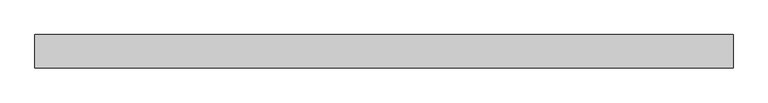
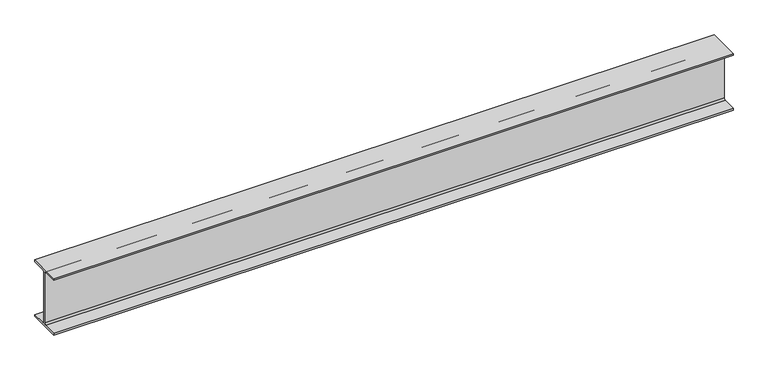
"""IFC4 building model written with IfcOpenShell, lengths in millimetres: beam geometry, Steel Beam_H-KSD3502 : H_SB_ASB_H-200x200x8x12."""

import ifcopenshell
import ifcopenshell.guid

model = None  # the IFC model being written
_history = None  # IfcOwnerHistory: only IFC2X3 demands one
_inside = {}  # id of a spatial element -> (the spatial element, [elements in it])
_under = {}  # id of a project, library or spatial element -> (it, [spatial elements below it])
_declared = {}  # id of a project -> (the project, [libraries it declares])
_typed = {}  # id of a type object -> (the type object, [elements of that type])
_made_of = {}  # id of a material, layer set ... -> (it, [elements and type objects made of it])


def new_model(schema):
    """Start an empty IFC model of exactly this schema.

    Asked for "IFC4X3", IfcOpenShell would pick the latest addendum, in which some entities
    have other attributes; the version numbers below select the first issue.
    IFC2X3 requires an IfcOwnerHistory on every rooted entity: one is made here for all.
    """
    global model, _history
    if schema == "IFC4X3":
        model = ifcopenshell.file(schema_version=(4, 3, 0, 0))
    else:
        model = ifcopenshell.file(schema=schema)
    _inside.clear()
    _under.clear()
    _declared.clear()
    _typed.clear()
    _made_of.clear()
    _history = None
    if model.schema == "IFC2X3":
        org = make("IfcOrganization", Name="unknown")
        user = make(
            "IfcPersonAndOrganization",
            ThePerson=make("IfcPerson", FamilyName="unknown"),
            TheOrganization=org,
        )
        app = make(
            "IfcApplication",
            ApplicationDeveloper=org,
            Version="unknown",
            ApplicationFullName="unknown",
            ApplicationIdentifier="unknown",
        )
        _history = make(
            "IfcOwnerHistory",
            OwningUser=user,
            OwningApplication=app,
            ChangeAction="ADDED",
            CreationDate=0,
        )
    return model


def make(cls, **values):
    """One entity of the class cls with the attributes given. An attribute that is None is left unset."""
    return model.create_entity(
        cls, **{name: value for name, value in values.items() if value is not None}
    )


def rooted(cls, **values):
    """An entity with a GlobalId (a new one), such as an element, a storey or a relation."""
    return make(cls, GlobalId=ifcopenshell.guid.new(), OwnerHistory=_history, **values)


def si_unit(unit_type, name, prefix=None):
    """IfcSIUnit, for example si_unit("LENGTHUNIT", "METRE", prefix="MILLI")."""
    return make("IfcSIUnit", UnitType=unit_type, Prefix=prefix, Name=name)


def assignment(units):
    """IfcUnitAssignment: the units of a project."""
    return None if units is None else make("IfcUnitAssignment", Units=units)


def point(xyz):
    """IfcCartesianPoint."""
    return None if xyz is None else make("IfcCartesianPoint", Coordinates=xyz)


def direction(xyz):
    """IfcDirection."""
    return None if xyz is None else make("IfcDirection", DirectionRatios=xyz)


def frame(location, z_axis=None, x_axis=None):
    """IfcAxis2Placement3D, a coordinate frame: its origin and axes. An axis left out is left unset."""
    return make(
        "IfcAxis2Placement3D",
        Location=point(location),
        Axis=direction(z_axis),
        RefDirection=direction(x_axis),
    )


def frame_2d(location, x_axis=None):
    """IfcAxis2Placement2D, a coordinate frame in the plane: its origin and x axis."""
    return make(
        "IfcAxis2Placement2D", Location=point(location), RefDirection=direction(x_axis)
    )


def origin():
    """The frame at (0, 0, 0) with its axes left unset."""
    return frame((0.0, 0.0, 0.0))


def place(relative_to, where):
    """IfcLocalPlacement: puts the frame where relative to a parent placement (None: the world)."""
    return make(
        "IfcLocalPlacement", PlacementRelTo=relative_to, RelativePlacement=where
    )


def context(
    kind, dimensions, precision=None, world=None, true_north=None, identifier=None
):
    """IfcGeometricRepresentationContext, for example the 3D "Model" context."""
    return make(
        "IfcGeometricRepresentationContext",
        ContextIdentifier=identifier,
        ContextType=kind,
        CoordinateSpaceDimension=dimensions,
        Precision=precision,
        WorldCoordinateSystem=world,
        TrueNorth=true_north,
    )


def project(units=None, contexts=None):
    """IfcProject with its units and contexts."""
    return rooted(
        "IfcProject",
        Name="project",
        RepresentationContexts=contexts,
        UnitsInContext=assignment(units),
    )


def spatial(cls, under=None, at=None, **own):
    """A site, building, storey or space (cls), placed at a placement, below another one or the project."""
    s = rooted(cls, ObjectPlacement=at, **own)
    if under is not None:
        _under.setdefault(under.id(), (under, []))[1].append(s)
    return s


def polyline(points):
    """IfcPolyline through the points."""
    return make("IfcPolyline", Points=[point(p) for p in points])


def circle_curve(where, radius):
    """IfcCircle in the frame where."""
    return make("IfcCircle", Position=where, Radius=radius)


def trimmed(basis, trim1, trim2, sense, master):
    """IfcTrimmedCurve: the piece of a basis curve between two trims."""
    return make(
        "IfcTrimmedCurve",
        BasisCurve=basis,
        Trim1=trim1,
        Trim2=trim2,
        SenseAgreement=sense,
        MasterRepresentation=master,
    )


def segment(curve, same_sense, transition):
    """IfcCompositeCurveSegment."""
    return make(
        "IfcCompositeCurveSegment",
        Transition=transition,
        SameSense=same_sense,
        ParentCurve=curve,
    )


def composite_curve(segments, self_intersect=None):
    """IfcCompositeCurve: segments joined end to end."""
    return make("IfcCompositeCurve", Segments=segments, SelfIntersect=self_intersect)


def outline(outer, holes=None, kind="AREA"):
    """IfcArbitraryClosedProfileDef: a profile drawn as a closed curve; with holes, ...WithVoids."""
    if holes is None:
        return make("IfcArbitraryClosedProfileDef", ProfileType=kind, OuterCurve=outer)
    return make(
        "IfcArbitraryProfileDefWithVoids",
        ProfileType=kind,
        OuterCurve=outer,
        InnerCurves=holes,
    )


def extrude(swept, where, along, depth):
    """IfcExtrudedAreaSolid: the profile swept, set in the frame where, extruded along a direction by depth."""
    return make(
        "IfcExtrudedAreaSolid",
        SweptArea=swept,
        Position=where,
        ExtrudedDirection=direction(along),
        Depth=depth,
    )


def shape(context_of_items, identifier, shape_type, items):
    """IfcShapeRepresentation: the items that make up one representation, for example the "Body"."""
    return make(
        "IfcShapeRepresentation",
        ContextOfItems=context_of_items,
        RepresentationIdentifier=identifier,
        RepresentationType=shape_type,
        Items=items,
    )


def source(mapping_origin, context_of_items, identifier, shape_type, items):
    """IfcRepresentationMap: a shape defined once, which mapped items show again and again."""
    return make(
        "IfcRepresentationMap",
        MappingOrigin=mapping_origin,
        MappedRepresentation=shape(context_of_items, identifier, shape_type, items),
    )


def transform(
    local_origin,
    x_axis=None,
    y_axis=None,
    z_axis=None,
    scale=None,
    scale2=None,
    scale3=None,
    uniform=True,
):
    """IfcCartesianTransformationOperator3D, or its non-uniform kind. x_axis, y_axis, z_axis: its Axis1, 2, 3."""
    if uniform:
        return make(
            "IfcCartesianTransformationOperator3D",
            Axis1=direction(x_axis),
            Axis2=direction(y_axis),
            LocalOrigin=point(local_origin),
            Scale=scale,
            Axis3=direction(z_axis),
        )
    return make(
        "IfcCartesianTransformationOperator3DnonUniform",
        Axis1=direction(x_axis),
        Axis2=direction(y_axis),
        LocalOrigin=point(local_origin),
        Scale=scale,
        Axis3=direction(z_axis),
        Scale2=scale2,
        Scale3=scale3,
    )


def mapped(mapping_source, mapping_target):
    """IfcMappedItem: shows the shape of a source again, moved by a transform."""
    return make(
        "IfcMappedItem", MappingSource=mapping_source, MappingTarget=mapping_target
    )


def made_of(thing, what):
    """Note that an element or type object is made of a material, layer set ...; save() writes the relation."""
    if what is not None:
        _made_of.setdefault(what.id(), (what, []))[1].append(thing)
    return thing


def element(
    cls,
    number,
    at=None,
    inside=None,
    cuts=None,
    type_object=None,
    material=None,
    context=None,
    identifier="Body",
    shape_type=None,
    held_by="IfcProductDefinitionShape",
    body=None,
    shapes=None,
    **own,
):
    """One element of the class cls, such as IfcWall. Its Tag is "e" and its number.

    at: its placement. inside: the storey or other place that contains it. cuts: it is an
    opening in that element (IfcRelVoidsElement). A single representation is given by context,
    identifier, shape_type and body (its items); several are given by shapes. held_by: the class
    of the entity that holds the representations. save() writes the other relations.
    """
    e = rooted(cls, Tag="e%d" % number, ObjectPlacement=at, **own)
    if body is not None:
        shapes = [shape(context, identifier, shape_type, body)]
    if shapes is not None:
        e.Representation = make(held_by, Representations=shapes)
    if inside is not None:
        _inside.setdefault(inside.id(), (inside, []))[1].append(e)
    if cuts is not None:
        rooted(
            "IfcRelVoidsElement", RelatingBuildingElement=cuts, RelatedOpeningElement=e
        )
    if type_object is not None:
        _typed.setdefault(type_object.id(), (type_object, []))[1].append(e)
    return made_of(e, material)


def aggregate(whole, parts):
    """IfcRelAggregates: a whole, such as a stair, and the parts it consists of."""
    return rooted("IfcRelAggregates", RelatingObject=whole, RelatedObjects=parts)


def save(model, path):
    """Write the relations noted so far, then the file.

    IfcRelAggregates (storeys below a building ...), IfcRelContainedInSpatialStructure (elements
    in a storey), IfcRelDefinesByType, IfcRelAssociatesMaterial and IfcRelDeclares: one each for
    every whole, place, type object, material and project.
    """
    for whole, parts in _under.values():
        aggregate(whole, parts)
    for where, things in _inside.values():
        rooted(
            "IfcRelContainedInSpatialStructure",
            RelatedElements=things,
            RelatingStructure=where,
        )
    for kind, things in _typed.values():
        rooted("IfcRelDefinesByType", RelatedObjects=things, RelatingType=kind)
    for what, things in _made_of.values():
        rooted("IfcRelAssociatesMaterial", RelatedObjects=things, RelatingMaterial=what)
    for by, libraries in _declared.values():
        rooted("IfcRelDeclares", RelatingContext=by, RelatedDefinitions=libraries)
    model.write(path)


def beam_b71a2e39(model_context):
    return source(origin(), model_context, "Body", "SweptSolid", [
        extrude(outline(composite_curve([segment(polyline([(82.5, -141.5), (82.5, -151.7), (-82.5, -151.7), (-82.5, -141.5), (-11.9, -141.5)]), True, "CONTINUOUS"), segment(trimmed(circle_curve(frame_2d((-11.9, -132.6)), 8.9), [point((-11.9, -141.5))], [point((-3.0, -132.6))], True, "CARTESIAN"), True, "CONTINUOUS"), segment(polyline([(-3.0, -132.6), (-3.0, 132.6)]), True, "CONTINUOUS"), segment(trimmed(circle_curve(frame_2d((-11.9, 132.6)), 8.9), [point((-3.0, 132.6))], [point((-11.9, 141.5))], True, "CARTESIAN"), True, "CONTINUOUS"), segment(polyline([(-11.9, 141.5), (-82.5, 141.5), (-82.5, 151.7), (82.5, 151.7), (82.5, 141.5), (11.9, 141.5)]), True, "CONTINUOUS"), segment(trimmed(circle_curve(frame_2d((11.9, 132.6)), 8.9), [point((11.9, 141.5))], [point((3.0, 132.6))], True, "CARTESIAN"), True, "CONTINUOUS"), segment(polyline([(3.0, 132.6), (3.0, -132.6)]), True, "CONTINUOUS"), segment(trimmed(circle_curve(frame_2d((11.9, -132.6)), 8.9), [point((3.0, -132.6))], [point((11.9, -141.5))], True, "CARTESIAN"), True, "CONTINUOUS"), segment(polyline([(11.9, -141.5), (82.5, -141.5)]), True, "CONTINUOUS")], self_intersect=False)), frame((-1683.7594404, 0.0, 0.0), z_axis=(1.0, 0.0, 0.0), x_axis=(0.0, 1.0, 0.0)), (0.0, 0.0, 1.0), 3450.380526),
    ])


if __name__ == "__main__":
    model = new_model("IFC4")
    model_context = context("Model", 3, world=origin())
    ifc_project = project(units=[si_unit("LENGTHUNIT", "METRE", prefix="MILLI")], contexts=[model_context])
    site = spatial("IfcSite", under=ifc_project)
    building = spatial("IfcBuilding", under=site)
    placement = place(None, origin())
    beam_shape = beam_b71a2e39(model_context)
    element("IfcBeam", 1, ObjectType="Steel Beam_H-KSD3502 : H_SB_ASB_H-200x200x8x12", at=placement, inside=building, context=model_context, shape_type="MappedRepresentation", body=[
        mapped(beam_shape, transform((0.0, 0.0, 0.0), x_axis=(1.0, 0.0, 0.0), y_axis=(0.0, 1.0, 0.0), z_axis=(0.0, 0.0, 1.0))),
    ])
    save(model, "model.ifc")

# Revit data of these elements
# Type "Steel Beam_H-KSD3502 : H_SB_ASB_H-200x200x8x12"
#   Width = 20.0 cm
#   Web Thickness = 0.8 cm
#   Web Fillet = 1.3 cm
#   Warping Constant = 141376.0 cm⁶
#   Torsional Moment of Inertia = 26.2485 cm⁴
#   Torsional Modulus = 1.0 cm³
#   Section Area = 63.53 cm²
#   Plastic Modulus weak axis = 244.0 cm³
#   Plastic Modulus strong axis = 525.0 cm³
#   Perimeter = 1.16 m²/m
#   Nominal Weight = 49.90 kgf/m
#   Moment of Inertia weak axis = 1600.00 cm⁴
#   Moment of Inertia strong axis = 4720.00 cm⁴
#   Height = 20.0 cm
#   Flange Thickness = 1.2 cm
#   Elastic Modulus weak axis = 160.0 cm³
#   Elastic Modulus strong axis = 472.0 cm³
#   Centroid Vertical = 10.0 cm
#   Centroid Horizontal = 10.0 cm
#   Length [instance default] = 1.5240 m
#   Structural Material [instance default] = Steel, 45-345
#   Assembly Code = ""
# Element 1 (IfcBeam, "Steel Beam_H-KSD3502 : H_SB_ASB_H-200x200x8x12")
#   Structural Material = none
# Materials
#   "Steel, 45-345": class "Metal", colour RGB 189 187 185, transparency 0, Description = "Steel 345 MPa", Cost = 0
